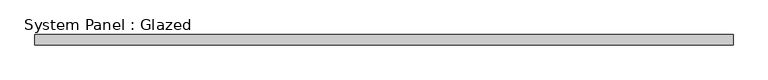
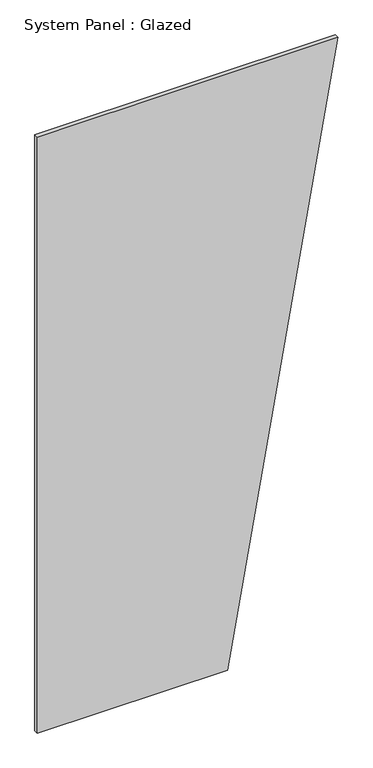
"""IFC4 building model written with IfcOpenShell, lengths in millimetres: plate geometry, System Panel : Glazed."""

from ifc_helpers import new_model, si_unit, frame, origin, place, context, project, spatial, polyline, outline, extrude, source, transform, mapped, element, save


def system_panel_glazed_d54edbd1(model_context):
    return source(origin(), model_context, "Body", "SweptSolid", [
        extrude(outline(polyline([(0.0, -873.5917397), (0.0, 231.112342), (3657.6, 873.5917397), (3657.6, -873.5917397), (0.0, -873.5917397)])), frame((0.0, -44.45, 0.0), z_axis=(0.0, 1.0, 0.0), x_axis=(0.0, 0.0, 1.0)), (0.0, 0.0, 1.0), 25.4),
    ])


if __name__ == "__main__":
    model = new_model("IFC4")
    model_context = context("Model", 3, world=origin())
    ifc_project = project(units=[si_unit("LENGTHUNIT", "METRE", prefix="MILLI")], contexts=[model_context])
    site = spatial("IfcSite", under=ifc_project)
    building = spatial("IfcBuilding", under=site)
    placement = place(None, origin())
    system_panel_glazed_shape = system_panel_glazed_d54edbd1(model_context)
    element("IfcPlate", 1, ObjectType="System Panel : Glazed", at=placement, inside=building, context=model_context, shape_type="MappedRepresentation", body=[
        mapped(system_panel_glazed_shape, transform((0.0, 0.0, 0.0), x_axis=(1.0, 0.0, 0.0), y_axis=(0.0, 1.0, 0.0), z_axis=(0.0, 0.0, 1.0))),
    ])
    save(model, "model.ifc")

# Revit data of these elements
# Type "System Panel : Glazed"
#   Construction Type Id = "GSP4R"
#   Analytic Construction = "1/8 in Pilkington single glazing"
#   Visual Light Transmittance = 0.9
#   Solar Heat Gain Coefficient = 0.86
#   Heat Transfer Coefficient (U) = 1.18115 BTU/(h·ft²·°F)
#   Define Thermal Properties by = 1
# Element 1 (IfcPlate, "System Panel : Glazed")
#   Materials on its faces: "Glass"
# Materials
#   "Glass": class "Glass", colour RGB 0 128 192, transparency 0.75, Description = "Soda Lime Glass", Cost = 0
